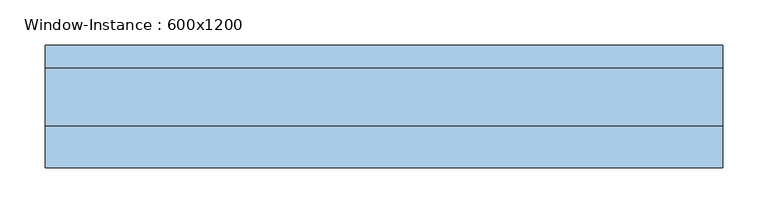
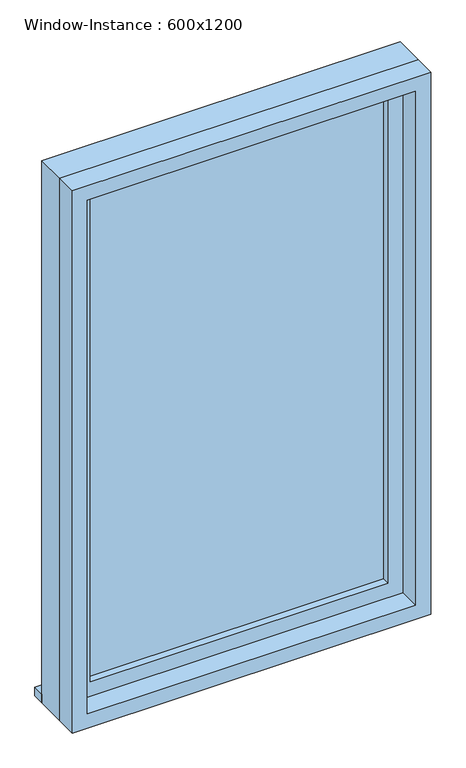
"""IFC4 building model written with IfcOpenShell, lengths in millimetres: window geometry, Window-Instance : 600x1200."""

from ifc_helpers import new_model, si_unit, frame, origin, place, context, project, spatial, polyline, outline, extrude, source, transform, mapped, element, save


def window_instance_600x1200_a370a862(model_context):
    return source(origin(), model_context, "Body", "SweptSolid", [
        extrude(outline(polyline([(-413.1, 80.4), (336.9, 80.4), (336.9, 55.0), (-413.1, 55.0), (-413.1, 80.4)])), frame((0.0, 0.0, 900.0), z_axis=(0.0, 0.0, 1.0), x_axis=(1.0, 0.0, 0.0)), (0.0, 0.0, 1.0), 19.05),
        extrude(outline(polyline([(273.4, 6.425), (-349.6, 6.425), (-349.6, 19.125), (273.4, 19.125), (273.4, 6.425)])), frame((0.0, 0.0, 963.5), z_axis=(0.0, 0.0, 1.0), x_axis=(1.0, 0.0, 0.0)), (0.0, 0.0, 1.0), 1073.0),
        extrude(outline(polyline([(2080.95, -394.05), (919.05, -394.05), (919.05, 317.85), (2080.95, 317.85), (2080.95, -394.05)]), holes=[polyline([(2036.5, -349.6), (2036.5, 273.4), (963.5, 273.4), (963.5, -349.6), (2036.5, -349.6)])]), frame((0.0, -9.45, 0.0), z_axis=(0.0, 1.0, 0.0), x_axis=(0.0, 0.0, 1.0)), (0.0, 0.0, 1.0), 44.45),
        extrude(outline(polyline([(2100.0, -413.1), (900.0, -413.1), (900.0, 336.9), (2100.0, 336.9), (2100.0, -413.1)]), holes=[polyline([(2068.25, -381.35), (2068.25, 305.15), (931.75, 305.15), (931.75, -381.35), (2068.25, -381.35)])]), frame((0.0, -55.0, 0.0), z_axis=(0.0, 1.0, 0.0), x_axis=(0.0, 0.0, 1.0)), (0.0, 0.0, 1.0), 45.55),
        extrude(outline(polyline([(2100.0, 336.9), (2100.0, -413.1), (900.0, -413.1), (900.0, 336.9), (2100.0, 336.9)]), holes=[polyline([(2080.95, 317.85), (919.05, 317.85), (919.05, -394.05), (2080.95, -394.05), (2080.95, 317.85)])]), frame((0.0, -9.45, 0.0), z_axis=(0.0, 1.0, 0.0), x_axis=(0.0, 0.0, 1.0)), (0.0, 0.0, 1.0), 64.45),
    ])


if __name__ == "__main__":
    model = new_model("IFC4")
    model_context = context("Model", 3, world=origin())
    ifc_project = project(units=[si_unit("LENGTHUNIT", "METRE", prefix="MILLI")], contexts=[model_context])
    site = spatial("IfcSite", under=ifc_project)
    building = spatial("IfcBuilding", under=site)
    placement = place(None, origin())
    window_instance_600x1200_shape = window_instance_600x1200_a370a862(model_context)
    element("IfcWindow", 1, ObjectType="Window-Instance : 600x1200", at=placement, inside=building, context=model_context, shape_type="MappedRepresentation", body=[
        mapped(window_instance_600x1200_shape, transform((0.0, 0.0, 0.0), x_axis=(1.0, 0.0, 0.0), y_axis=(0.0, 1.0, 0.0), z_axis=(0.0, 0.0, 1.0))),
    ])
    save(model, "model.ifc")

# Revit data of these elements
# Type "Window-Instance : 600x1200"
#   Type Mark = "7"
#   Construction Type Id = "GSP4R"
#   Assembly Code = "B2020100"
#   Analytic Construction = "1/8 in Pilkington single glazing"
#   Visual Light Transmittance = 0.9
#   Thermal Resistance (R) = 0.149095 (m²·K)/W
#   Solar Heat Gain Coefficient = 0.86
#   Heat Transfer Coefficient (U) = 6.70716 W/(m²·K)
#   Height [instance default] = 1200 mm
#   Default Sill Height = 900 mm
#   Width [instance default] = 600 mm
#   Window Inset = 20 mm
#   Glass Pane Material = WW-EC-GL-Storefront
#   Sash Material = WW-EC-RGB-White
#   Wall Closure = (empty or 0)
# Element 1 (IfcWindow, "Window-Instance : 600x1200")
#   Width = 750 mm
#   Materials on its faces: "WW-EC-RGB-White", "WW-EC-GL-Storefront"
# Materials
#   "WW-EC-GL-Storefront": class "Glass", colour RGB 236 240 239, transparency 0.85, Description = "Storefront Glass", Cost = 0
#   "WW-EC-RGB-White": class "Generic", colour RGB 255 255 255, transparency 0, Comments = "If region requests off-white, swith asset color to RGB 231-228-220", Description = "Generic Color", Cost = 0
